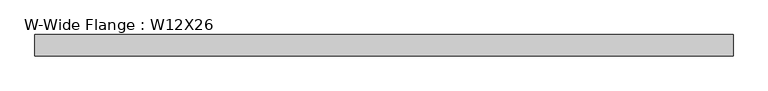
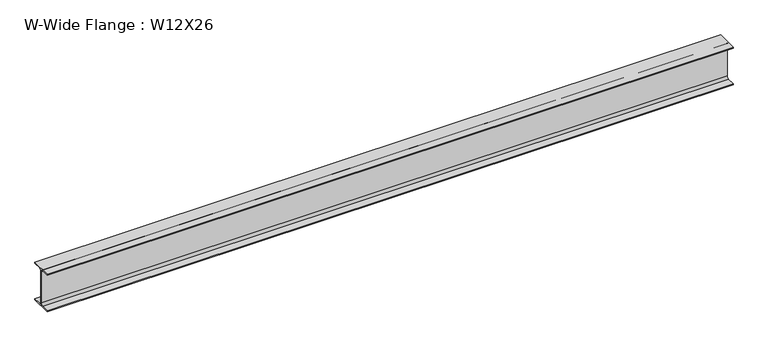
"""IFC4 building model written with IfcOpenShell, lengths in millimetres: beam geometry, W-Wide Flange : W12X26."""

import ifcopenshell
import ifcopenshell.guid

model = None  # the IFC model being written
_history = None  # IfcOwnerHistory: only IFC2X3 demands one
_inside = {}  # id of a spatial element -> (the spatial element, [elements in it])
_under = {}  # id of a project, library or spatial element -> (it, [spatial elements below it])
_declared = {}  # id of a project -> (the project, [libraries it declares])
_typed = {}  # id of a type object -> (the type object, [elements of that type])
_made_of = {}  # id of a material, layer set ... -> (it, [elements and type objects made of it])


def new_model(schema):
    """Start an empty IFC model of exactly this schema.

    Asked for "IFC4X3", IfcOpenShell would pick the latest addendum, in which some entities
    have other attributes; the version numbers below select the first issue.
    IFC2X3 requires an IfcOwnerHistory on every rooted entity: one is made here for all.
    """
    global model, _history
    if schema == "IFC4X3":
        model = ifcopenshell.file(schema_version=(4, 3, 0, 0))
    else:
        model = ifcopenshell.file(schema=schema)
    _inside.clear()
    _under.clear()
    _declared.clear()
    _typed.clear()
    _made_of.clear()
    _history = None
    if model.schema == "IFC2X3":
        org = make("IfcOrganization", Name="unknown")
        user = make(
            "IfcPersonAndOrganization",
            ThePerson=make("IfcPerson", FamilyName="unknown"),
            TheOrganization=org,
        )
        app = make(
            "IfcApplication",
            ApplicationDeveloper=org,
            Version="unknown",
            ApplicationFullName="unknown",
            ApplicationIdentifier="unknown",
        )
        _history = make(
            "IfcOwnerHistory",
            OwningUser=user,
            OwningApplication=app,
            ChangeAction="ADDED",
            CreationDate=0,
        )
    return model


def make(cls, **values):
    """One entity of the class cls with the attributes given. An attribute that is None is left unset."""
    return model.create_entity(
        cls, **{name: value for name, value in values.items() if value is not None}
    )


def rooted(cls, **values):
    """An entity with a GlobalId (a new one), such as an element, a storey or a relation."""
    return make(cls, GlobalId=ifcopenshell.guid.new(), OwnerHistory=_history, **values)


def si_unit(unit_type, name, prefix=None):
    """IfcSIUnit, for example si_unit("LENGTHUNIT", "METRE", prefix="MILLI")."""
    return make("IfcSIUnit", UnitType=unit_type, Prefix=prefix, Name=name)


def assignment(units):
    """IfcUnitAssignment: the units of a project."""
    return None if units is None else make("IfcUnitAssignment", Units=units)


def point(xyz):
    """IfcCartesianPoint."""
    return None if xyz is None else make("IfcCartesianPoint", Coordinates=xyz)


def direction(xyz):
    """IfcDirection."""
    return None if xyz is None else make("IfcDirection", DirectionRatios=xyz)


def frame(location, z_axis=None, x_axis=None):
    """IfcAxis2Placement3D, a coordinate frame: its origin and axes. An axis left out is left unset."""
    return make(
        "IfcAxis2Placement3D",
        Location=point(location),
        Axis=direction(z_axis),
        RefDirection=direction(x_axis),
    )


def frame_2d(location, x_axis=None):
    """IfcAxis2Placement2D, a coordinate frame in the plane: its origin and x axis."""
    return make(
        "IfcAxis2Placement2D", Location=point(location), RefDirection=direction(x_axis)
    )


def origin():
    """The frame at (0, 0, 0) with its axes left unset."""
    return frame((0.0, 0.0, 0.0))


def place(relative_to, where):
    """IfcLocalPlacement: puts the frame where relative to a parent placement (None: the world)."""
    return make(
        "IfcLocalPlacement", PlacementRelTo=relative_to, RelativePlacement=where
    )


def context(
    kind, dimensions, precision=None, world=None, true_north=None, identifier=None
):
    """IfcGeometricRepresentationContext, for example the 3D "Model" context."""
    return make(
        "IfcGeometricRepresentationContext",
        ContextIdentifier=identifier,
        ContextType=kind,
        CoordinateSpaceDimension=dimensions,
        Precision=precision,
        WorldCoordinateSystem=world,
        TrueNorth=true_north,
    )


def project(units=None, contexts=None):
    """IfcProject with its units and contexts."""
    return rooted(
        "IfcProject",
        Name="project",
        RepresentationContexts=contexts,
        UnitsInContext=assignment(units),
    )


def spatial(cls, under=None, at=None, **own):
    """A site, building, storey or space (cls), placed at a placement, below another one or the project."""
    s = rooted(cls, ObjectPlacement=at, **own)
    if under is not None:
        _under.setdefault(under.id(), (under, []))[1].append(s)
    return s


def polyline(points):
    """IfcPolyline through the points."""
    return make("IfcPolyline", Points=[point(p) for p in points])


def circle_curve(where, radius):
    """IfcCircle in the frame where."""
    return make("IfcCircle", Position=where, Radius=radius)


def trimmed(basis, trim1, trim2, sense, master):
    """IfcTrimmedCurve: the piece of a basis curve between two trims."""
    return make(
        "IfcTrimmedCurve",
        BasisCurve=basis,
        Trim1=trim1,
        Trim2=trim2,
        SenseAgreement=sense,
        MasterRepresentation=master,
    )


def segment(curve, same_sense, transition):
    """IfcCompositeCurveSegment."""
    return make(
        "IfcCompositeCurveSegment",
        Transition=transition,
        SameSense=same_sense,
        ParentCurve=curve,
    )


def composite_curve(segments, self_intersect=None):
    """IfcCompositeCurve: segments joined end to end."""
    return make("IfcCompositeCurve", Segments=segments, SelfIntersect=self_intersect)


def outline(outer, holes=None, kind="AREA"):
    """IfcArbitraryClosedProfileDef: a profile drawn as a closed curve; with holes, ...WithVoids."""
    if holes is None:
        return make("IfcArbitraryClosedProfileDef", ProfileType=kind, OuterCurve=outer)
    return make(
        "IfcArbitraryProfileDefWithVoids",
        ProfileType=kind,
        OuterCurve=outer,
        InnerCurves=holes,
    )


def extrude(swept, where, along, depth):
    """IfcExtrudedAreaSolid: the profile swept, set in the frame where, extruded along a direction by depth."""
    return make(
        "IfcExtrudedAreaSolid",
        SweptArea=swept,
        Position=where,
        ExtrudedDirection=direction(along),
        Depth=depth,
    )


def shape(context_of_items, identifier, shape_type, items):
    """IfcShapeRepresentation: the items that make up one representation, for example the "Body"."""
    return make(
        "IfcShapeRepresentation",
        ContextOfItems=context_of_items,
        RepresentationIdentifier=identifier,
        RepresentationType=shape_type,
        Items=items,
    )


def source(mapping_origin, context_of_items, identifier, shape_type, items):
    """IfcRepresentationMap: a shape defined once, which mapped items show again and again."""
    return make(
        "IfcRepresentationMap",
        MappingOrigin=mapping_origin,
        MappedRepresentation=shape(context_of_items, identifier, shape_type, items),
    )


def transform(
    local_origin,
    x_axis=None,
    y_axis=None,
    z_axis=None,
    scale=None,
    scale2=None,
    scale3=None,
    uniform=True,
):
    """IfcCartesianTransformationOperator3D, or its non-uniform kind. x_axis, y_axis, z_axis: its Axis1, 2, 3."""
    if uniform:
        return make(
            "IfcCartesianTransformationOperator3D",
            Axis1=direction(x_axis),
            Axis2=direction(y_axis),
            LocalOrigin=point(local_origin),
            Scale=scale,
            Axis3=direction(z_axis),
        )
    return make(
        "IfcCartesianTransformationOperator3DnonUniform",
        Axis1=direction(x_axis),
        Axis2=direction(y_axis),
        LocalOrigin=point(local_origin),
        Scale=scale,
        Axis3=direction(z_axis),
        Scale2=scale2,
        Scale3=scale3,
    )


def mapped(mapping_source, mapping_target):
    """IfcMappedItem: shows the shape of a source again, moved by a transform."""
    return make(
        "IfcMappedItem", MappingSource=mapping_source, MappingTarget=mapping_target
    )


def made_of(thing, what):
    """Note that an element or type object is made of a material, layer set ...; save() writes the relation."""
    if what is not None:
        _made_of.setdefault(what.id(), (what, []))[1].append(thing)
    return thing


def element(
    cls,
    number,
    at=None,
    inside=None,
    cuts=None,
    type_object=None,
    material=None,
    context=None,
    identifier="Body",
    shape_type=None,
    held_by="IfcProductDefinitionShape",
    body=None,
    shapes=None,
    **own,
):
    """One element of the class cls, such as IfcWall. Its Tag is "e" and its number.

    at: its placement. inside: the storey or other place that contains it. cuts: it is an
    opening in that element (IfcRelVoidsElement). A single representation is given by context,
    identifier, shape_type and body (its items); several are given by shapes. held_by: the class
    of the entity that holds the representations. save() writes the other relations.
    """
    e = rooted(cls, Tag="e%d" % number, ObjectPlacement=at, **own)
    if body is not None:
        shapes = [shape(context, identifier, shape_type, body)]
    if shapes is not None:
        e.Representation = make(held_by, Representations=shapes)
    if inside is not None:
        _inside.setdefault(inside.id(), (inside, []))[1].append(e)
    if cuts is not None:
        rooted(
            "IfcRelVoidsElement", RelatingBuildingElement=cuts, RelatedOpeningElement=e
        )
    if type_object is not None:
        _typed.setdefault(type_object.id(), (type_object, []))[1].append(e)
    return made_of(e, material)


def aggregate(whole, parts):
    """IfcRelAggregates: a whole, such as a stair, and the parts it consists of."""
    return rooted("IfcRelAggregates", RelatingObject=whole, RelatedObjects=parts)


def save(model, path):
    """Write the relations noted so far, then the file.

    IfcRelAggregates (storeys below a building ...), IfcRelContainedInSpatialStructure (elements
    in a storey), IfcRelDefinesByType, IfcRelAssociatesMaterial and IfcRelDeclares: one each for
    every whole, place, type object, material and project.
    """
    for whole, parts in _under.values():
        aggregate(whole, parts)
    for where, things in _inside.values():
        rooted(
            "IfcRelContainedInSpatialStructure",
            RelatedElements=things,
            RelatingStructure=where,
        )
    for kind, things in _typed.values():
        rooted("IfcRelDefinesByType", RelatedObjects=things, RelatingType=kind)
    for what, things in _made_of.values():
        rooted("IfcRelAssociatesMaterial", RelatedObjects=things, RelatingMaterial=what)
    for by, libraries in _declared.values():
        rooted("IfcRelDeclares", RelatingContext=by, RelatedDefinitions=libraries)
    model.write(path)


def w_wide_flange_w12x26_4d76a115(model_context):
    return source(origin(), model_context, "Body", "SweptSolid", [
        extrude(outline(composite_curve([segment(polyline([(82.4011719, -145.5539063), (82.4011719, -155.178125), (-82.4011719, -155.178125), (-82.4011719, -145.5539063), (-20.2902344, -145.5539063)]), True, "CONTINUOUS"), segment(trimmed(circle_curve(frame_2d((-20.2902344, -128.190625)), 17.3632812), [point((-20.2902344, -145.5539063))], [point((-2.9269531, -128.190625))], True, "CARTESIAN"), True, "CONTINUOUS"), segment(polyline([(-2.9269531, -128.190625), (-2.9269531, 128.190625)]), True, "CONTINUOUS"), segment(trimmed(circle_curve(frame_2d((-20.2902344, 128.190625)), 17.3632812), [point((-2.9269531, 128.190625))], [point((-20.2902344, 145.5539062))], True, "CARTESIAN"), True, "CONTINUOUS"), segment(polyline([(-20.2902344, 145.5539062), (-82.4011719, 145.5539062), (-82.4011719, 155.178125), (82.4011719, 155.178125), (82.4011719, 145.5539062), (20.2902344, 145.5539062)]), True, "CONTINUOUS"), segment(trimmed(circle_curve(frame_2d((20.2902344, 128.190625)), 17.3632812), [point((20.2902344, 145.5539062))], [point((2.9269531, 128.190625))], True, "CARTESIAN"), True, "CONTINUOUS"), segment(polyline([(2.9269531, 128.190625), (2.9269531, -128.190625)]), True, "CONTINUOUS"), segment(trimmed(circle_curve(frame_2d((20.2902344, -128.190625)), 17.3632812), [point((2.9269531, -128.190625))], [point((20.2902344, -145.5539063))], True, "CARTESIAN"), True, "CONTINUOUS"), segment(polyline([(20.2902344, -145.5539063), (82.4011719, -145.5539063)]), True, "CONTINUOUS")], self_intersect=False)), frame((-2667.0, 0.0, 0.0), z_axis=(1.0, 0.0, 0.0), x_axis=(0.0, 1.0, 0.0)), (0.0, 0.0, 1.0), 5334.0),
    ])


if __name__ == "__main__":
    model = new_model("IFC4")
    model_context = context("Model", 3, world=origin())
    ifc_project = project(units=[si_unit("LENGTHUNIT", "METRE", prefix="MILLI")], contexts=[model_context])
    site = spatial("IfcSite", under=ifc_project)
    building = spatial("IfcBuilding", under=site)
    placement = place(None, origin())
    w_wide_flange_w12x26_shape = w_wide_flange_w12x26_4d76a115(model_context)
    element("IfcBeam", 1, ObjectType="W-Wide Flange : W12X26", at=placement, inside=building, context=model_context, shape_type="MappedRepresentation", body=[
        mapped(w_wide_flange_w12x26_shape, transform((0.0, 0.0, 0.0), x_axis=(1.0, 0.0, 0.0), y_axis=(0.0, 1.0, 0.0), z_axis=(0.0, 0.0, 1.0))),
    ])
    save(model, "model.ifc")

# Revit data of these elements
# Type "W-Wide Flange : W12X26"
#   Assembly Code = "B10"
#   W = 26
#   Length [instance default] = 5' - 0"
#   bf = 0' - 6 125/256"
#   d = 1' - 0 7/32"
#   k = 0' - 1 1/16"
#   k2 = 0' - 0 175/256"
#   tf = 0' - 0 97/256"
#   tw = 0' - 0 59/256"
#   A = 0.053125 SF
#   Structural Material [instance default] = none
# Element 1 (IfcBeam, "W-Wide Flange : W12X26")
#   Structural Material = PAINTED STEEL
#   Materials on its faces: "PAINTED STEEL"
# Materials
#   "PAINTED STEEL": class "Generic", colour RGB 120 120 120, transparency 0, Cost = 0
